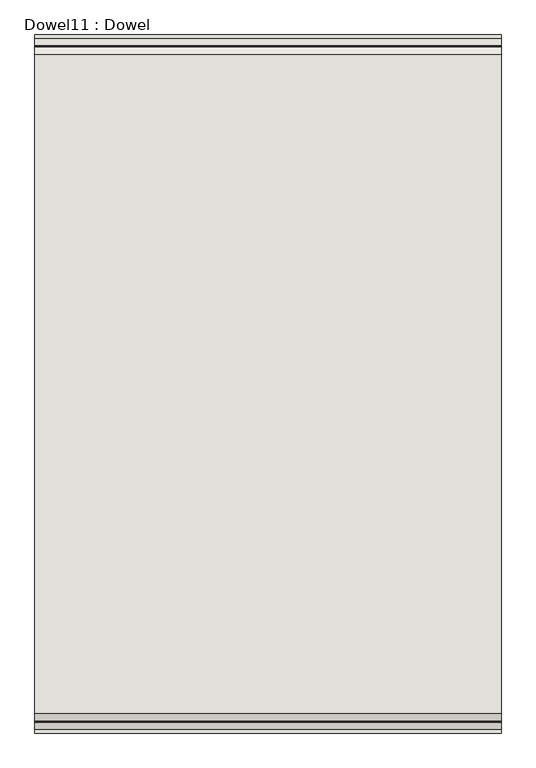
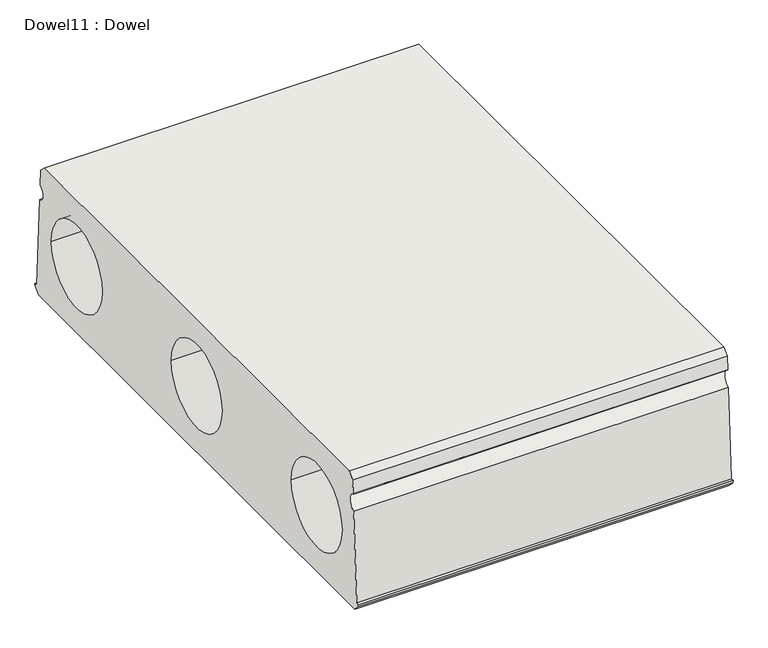
"""IFC4 building model written with IfcOpenShell, lengths in millimetres: wall geometry, Dowel11 : Dowel."""

from ifc_helpers import new_model, si_unit, point, frame, frame_2d, origin, place, context, project, spatial, polyline, circle_curve, trimmed, segment, composite_curve, outline, extrude, source, transform, mapped, element, save


def dowel11_dowel_5e8bf0fa(model_context):
    return source(origin(), model_context, "Body", "SweptSolid", [
        extrude(outline(composite_curve([segment(polyline([(-652.2998095, 2183.8462588), (494.5752653, 2183.8462588), (507.2752399, 2171.1462842), (509.1208332, 2134.8948264)]), True, "CONTINUOUS"), segment(trimmed(circle_curve(frame_2d((514.6427832, 2118.4686729)), 17.3294677), [point((509.1208332, 2134.8948264))], [point((511.3260506, 2101.4595655))], True, "CARTESIAN"), True, "CONTINUOUS"), segment(polyline([(511.3260506, 2101.4595655), (523.1502399, 1898.0462208), (529.1502279, 1898.0462208), (528.4502293, 1892.0462328), (515.4502553, 1879.0462588), (-673.1747995, 1879.0462588), (-686.1747735, 1892.0462328), (-686.8747721, 1898.0462208), (-680.8747841, 1898.0462208), (-669.0505948, 2101.4595655)]), True, "CONTINUOUS"), segment(trimmed(circle_curve(frame_2d((-675.4772325, 2120.8655788)), 20.4424809), [point((-669.0505948, 2101.4595655))], [point((-666.8453774, 2139.3962588))], True, "CARTESIAN"), True, "CONTINUOUS"), segment(polyline([(-666.8453774, 2139.3962588), (-664.9997841, 2171.1462842), (-652.2998095, 2183.8462588)]), True, "CONTINUOUS")], self_intersect=False), holes=[composite_curve([segment(trimmed(circle_curve(frame_2d((-529.7122721, 2031.4462588)), 95.25), [point((-624.9622721, 2031.4462588))], [point((-434.4622721, 2031.4462588))], True, "CARTESIAN"), True, "CONTINUOUS"), segment(trimmed(circle_curve(frame_2d((-529.7122721, 2031.4462588)), 95.25), [point((-434.4622721, 2031.4462588))], [point((-624.9622721, 2031.4462588))], True, "CARTESIAN"), True, "CONTINUOUS")], self_intersect=False), composite_curve([segment(trimmed(circle_curve(frame_2d((-78.8622721, 2031.4462588)), 95.25), [point((-174.1122721, 2031.4462588))], [point((16.3877279, 2031.4462588))], True, "CARTESIAN"), True, "CONTINUOUS"), segment(trimmed(circle_curve(frame_2d((-78.8622721, 2031.4462588)), 95.25), [point((16.3877279, 2031.4462588))], [point((-174.1122721, 2031.4462588))], True, "CARTESIAN"), True, "CONTINUOUS")], self_intersect=False), composite_curve([segment(trimmed(circle_curve(frame_2d((371.9877279, 2031.4462588)), 95.25), [point((276.7377279, 2031.4462588))], [point((467.2377279, 2031.4462588))], True, "CARTESIAN"), True, "CONTINUOUS"), segment(trimmed(circle_curve(frame_2d((371.9877279, 2031.4462588)), 95.25), [point((467.2377279, 2031.4462588))], [point((276.7377279, 2031.4462588))], True, "CARTESIAN"), True, "CONTINUOUS")], self_intersect=False)]), frame((375102.3526825, 0.0, 0.0), z_axis=(1.0, 0.0, 0.0), x_axis=(0.0, 1.0, 0.0)), (0.0, 0.0, 1.0), 812.8),
    ])


if __name__ == "__main__":
    model = new_model("IFC4")
    model_context = context("Model", 3, world=origin())
    ifc_project = project(units=[si_unit("LENGTHUNIT", "METRE", prefix="MILLI")], contexts=[model_context])
    site = spatial("IfcSite", under=ifc_project)
    building = spatial("IfcBuilding", under=site)
    placement = place(None, origin())
    dowel11_dowel_shape = dowel11_dowel_5e8bf0fa(model_context)
    element("IfcWall", 1, ObjectType="Dowel11 : Dowel", at=placement, inside=building, context=model_context, shape_type="MappedRepresentation", body=[
        mapped(dowel11_dowel_shape, transform((0.0, 0.0, 0.0), x_axis=(1.0, 0.0, 0.0), y_axis=(0.0, 1.0, 0.0), z_axis=(0.0, 0.0, 1.0))),
    ])
    save(model, "model.ifc")

# Revit data of these elements
# Element 1 (IfcWall, "Dowel11 : Dowel")
#   Materials on its faces: "PRECAST PLANK - SEE PRECAST SHOPS FOR SIZE"
# Materials
#   "PRECAST PLANK - SEE PRECAST SHOPS FOR SIZE": class "Concrete", colour RGB 191 191 191, transparency 0, Description = "Cast-in-place concrete", Cost = 0
